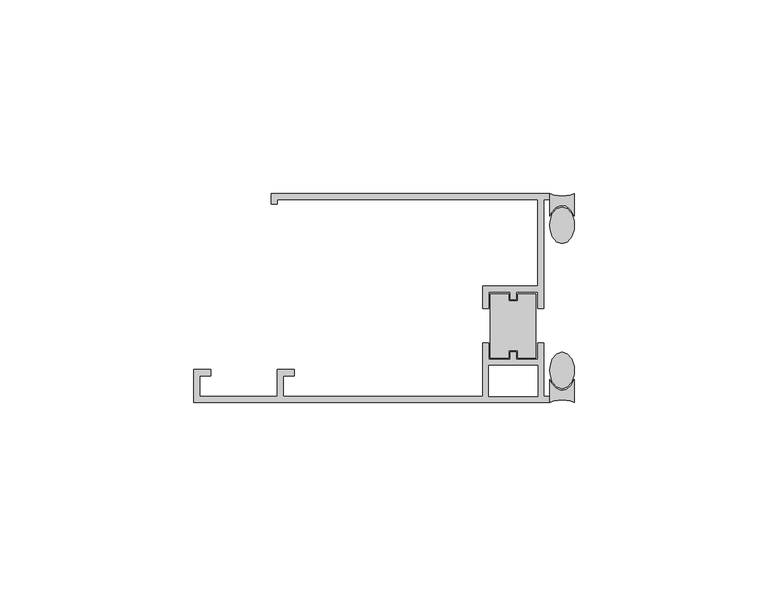
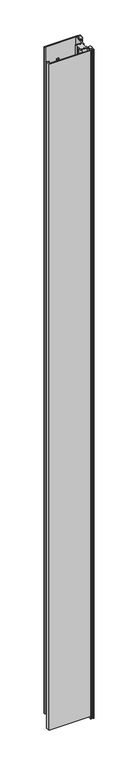
"""IFC4 building model written with IfcOpenShell, lengths in millimetres: proxy geometry, Generic Models 2:Generic Models 2:310765:Generic Models 2:310765 : Generic Models 2:Generic Models 2:310765:7 : Generic Models 2:Generic Models 2:310765:Generic Models 2:310765 : Generic Models 2:Generic Models 2:310765:300385."""

from ifc_helpers import new_model, si_unit, frame, origin, place, context, project, spatial, polyline, outline, extrude, source, transform, mapped, element, save


def generic_models_a9e8c91f(model_context):
    return source(origin(), model_context, "Body", "SweptSolid", [
        extrude(outline(polyline([(599957.7867239, -536507.0151803), (599958.1730415, -536507.8754613), (599959.256527, -536509.1850364), (599960.6067747, -536509.7853899), (599962.012551, -536509.582602), (599963.2539351, -536508.608397), (599964.1367239, -536507.0151803), (599964.1367239, -536512.8832724), (599963.1709607, -536512.5058638), (599960.9617239, -536512.1921777), (599958.7524872, -536512.5058638), (599957.7867239, -536512.8832724), (599957.7867239, -536507.0151803)])), frame((0.0, 0.0, 8511.4772069), z_axis=(0.0, 0.0, 1.0), x_axis=(1.0, 0.0, 0.0)), (0.0, 0.0, 1.0), 1539.6863224),
        extrude(outline(polyline([(599957.8663278, -536503.5917968), (599958.479409, -536501.6821825), (599959.5841431, -536500.3606885), (599960.9617239, -536499.8890527), (599962.3393048, -536500.3606885), (599963.4440389, -536501.6821825), (599964.0571201, -536503.5917968), (599964.1367239, -536504.6515527), (599964.0571201, -536505.7113086), (599963.4440389, -536507.6209229), (599962.3393048, -536508.9424169), (599960.9617239, -536509.4140527), (599959.5841431, -536508.9424169), (599958.479409, -536507.6209229), (599957.8663278, -536505.7113086), (599957.7867239, -536504.6515527), (599957.8663278, -536503.5917968)])), frame((0.0, 0.0, 8511.4772069), z_axis=(0.0, 0.0, 1.0), x_axis=(1.0, 0.0, 0.0)), (0.0, 0.0, 1.0), 1539.6863224),
        extrude(outline(polyline([(599959.5841431, -536462.8241279), (599960.9617239, -536462.3524921), (599962.3393048, -536462.8241279), (599963.4440389, -536464.1456219), (599964.0571201, -536466.0552361), (599964.1367239, -536467.1149921), (599964.0571201, -536468.174748), (599963.4440389, -536470.0843623), (599962.3393048, -536471.4058563), (599960.9617239, -536471.8774921), (599959.5841431, -536471.4058563), (599958.479409, -536470.0843623), (599957.8663278, -536468.174748), (599957.7867239, -536467.1149921), (599957.8663278, -536466.0552361), (599958.479409, -536464.1456219), (599959.5841431, -536462.8241279)])), frame((0.0, 0.0, 8511.4772069), z_axis=(0.0, 0.0, 1.0), x_axis=(1.0, 0.0, 0.0)), (0.0, 0.0, 1.0), 1539.6863224),
        extrude(outline(polyline([(599963.1709607, -536459.260681), (599964.1367239, -536458.8832724), (599964.1367239, -536464.7513645), (599963.2539351, -536463.1581478), (599962.012551, -536462.1839428), (599960.6067747, -536461.9811549), (599959.256527, -536462.5815084), (599958.1730415, -536463.8910835), (599957.7867239, -536464.7513645), (599957.7867239, -536458.8832724), (599958.7524872, -536459.260681), (599960.9617239, -536459.5743671), (599963.1709607, -536459.260681)])), frame((0.0, 0.0, 8511.4772069), z_axis=(0.0, 0.0, 1.0), x_axis=(1.0, 0.0, 0.0)), (0.0, 0.0, 1.0), 1539.6863224),
        extrude(outline(polyline([(599942.4386017, -536484.8160062), (599947.1361003, -536484.8160062), (599947.1361003, -536486.7414217), (599949.5173503, -536486.7414217), (599949.5173503, -536484.8160062), (599954.2148489, -536484.8160062), (599954.2148489, -536501.3682624), (599949.5173503, -536501.3682624), (599949.5173503, -536499.442847), (599947.1361003, -536499.442847), (599947.1361003, -536501.3682624), (599942.4386017, -536501.3682624), (599942.4386017, -536484.8160062)])), frame((0.0, 0.0, 8517.747603), z_axis=(0.0, 0.0, 1.0), x_axis=(1.0, 0.0, 0.0)), (0.0, 0.0, 1.0), 1533.4159263),
        extrude(outline(polyline([(599865.7867239, -536504.4369008), (599870.1740505, -536504.4369008), (599870.1740505, -536506.0244008), (599867.3742239, -536506.0244008), (599867.3742239, -536511.2957724), (599887.3742239, -536511.2957724), (599887.3742239, -536504.4369008), (599891.7615505, -536504.4369008), (599891.7615505, -536506.0244008), (599888.9617239, -536506.0244008), (599888.9617239, -536511.2957724), (599940.4542267, -536511.2957724), (599940.4542267, -536497.5979499), (599942.0417267, -536497.5979499), (599942.0417267, -536501.7651374), (599947.5329753, -536501.7651374), (599947.5329753, -536499.8397219), (599949.1204753, -536499.8397219), (599949.1204753, -536501.7651374), (599954.6117239, -536501.7651374), (599954.6117239, -536497.5979499), (599956.1992239, -536497.5979499), (599956.1992239, -536511.2957724), (599957.7867239, -536511.2957724), (599957.7867239, -536512.8832724), (599865.7867239, -536512.8832724), (599865.7867239, -536504.4369008)]), holes=[polyline([(599942.0417267, -536511.2957724), (599954.6117239, -536511.2957724), (599954.6117239, -536503.3526374), (599942.0417267, -536503.3526374), (599942.0417267, -536511.2957724)])]), frame((0.0, 0.0, 8517.747603), z_axis=(0.0, 0.0, 1.0), x_axis=(1.0, 0.0, 0.0)), (0.0, 0.0, 1.0), 1533.4159263),
        extrude(outline(polyline([(599957.7867239, -536460.4707724), (599956.1992239, -536460.4707724), (599956.1992239, -536488.5863187), (599954.6117239, -536488.5863187), (599954.6117239, -536484.4191312), (599949.1204753, -536484.4191312), (599949.1204753, -536486.3445467), (599947.5329753, -536486.3445467), (599947.5329753, -536484.4191312), (599942.0417267, -536484.4191312), (599942.0417267, -536488.5863187), (599940.4542267, -536488.5863187), (599940.4542267, -536482.8316312), (599954.6117239, -536482.8316312), (599954.6117239, -536460.4707724), (599887.3742239, -536460.4707724), (599887.3742239, -536461.5983623), (599885.7867239, -536461.5983623), (599885.7867239, -536458.8832724), (599957.7867239, -536458.8832724), (599957.7867239, -536460.4707724)])), frame((0.0, 0.0, 8517.747603), z_axis=(0.0, 0.0, 1.0), x_axis=(1.0, 0.0, 0.0)), (0.0, 0.0, 1.0), 1533.4159263),
    ])


if __name__ == "__main__":
    model = new_model("IFC4")
    model_context = context("Model", 3, world=origin())
    ifc_project = project(units=[si_unit("LENGTHUNIT", "METRE", prefix="MILLI")], contexts=[model_context])
    site = spatial("IfcSite", under=ifc_project)
    building = spatial("IfcBuilding", under=site)
    placement = place(None, origin())
    generic_models_shape = generic_models_a9e8c91f(model_context)
    element("IfcBuildingElementProxy", 1, Name="Generic Models 2:Generic Models 2:310765:Generic Models 2:310765 : Generic Models 2:Generic Models 2:310765:7 : Generic Models 2:Generic Models 2:310765:Generic Models 2:310765 : Generic Models 2:Generic Models 2:310765:300385", ObjectType="Generic Models 2:Generic Models 2:310765:Generic Models 2:310765 : Generic Models 2:Generic Models 2:310765:7 : Generic Models 2:Generic Models 2:310765:Generic Models 2:310765 : Generic Models 2:Generic Models 2:310765:300385", at=placement, inside=building, context=model_context, shape_type="MappedRepresentation", body=[
        mapped(generic_models_shape, transform((0.0, 0.0, 0.0), x_axis=(1.0, 0.0, 0.0), y_axis=(0.0, 1.0, 0.0), z_axis=(0.0, 0.0, 1.0))),
    ])
    save(model, "model.ifc")

# Revit data of these elements
# Type "Generic Models 2:Generic Models 2:310765:Generic Models 2:310765 : Generic Models 2:Generic Models 2:310765:7 : Generic Models 2:Generic Models 2:310765:Generic Models 2:310765 : Generic Models 2:Generic Models 2:310765:300385"
#   NameOverride = "Generic Models 2:Generic Models 2:310765:Generic Models 2:310765 : Generic Models 2:Generic Models 2:310765:300385"
#   ObjectTypeOverride = "Generic Models 2:310765 : Generic Models 2:Generic Models 2:310765"
#   Reference = "Generic Models 2"
#   Tag = "300385"
# Element 1 (IfcBuildingElementProxy, "Generic Models 2:Generic Models 2:310765:Generic Models 2:310765 : Generic Models 2:Generic Models 2:310765:7 : Generic Models 2:Generic Models 2:310765:Generic Models 2:310765 : Generic Models 2:Generic Models 2:310765:300385")
#   Materials on its faces: "SEALANT & BACKER ROD", "THERMAL BROKEN ALUMINUM STOREFRONT FOR POLYCARBONATE"
# Materials
#   "SEALANT & BACKER ROD": class "Unassigned", colour RGB 120 120 120, transparency 0, Cost = 0
#   "THERMAL BROKEN ALUMINUM STOREFRONT FOR POLYCARBONATE": class "Unassigned", colour RGB 244 244 244, transparency 0, Keynote = "M07611300.01", Cost = 0
